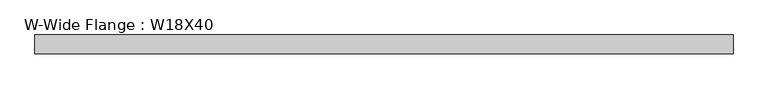
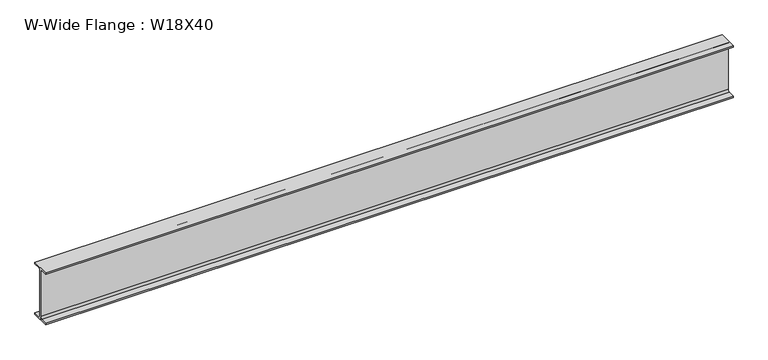
"""IFC4 building model written with IfcOpenShell, lengths in millimetres: beam geometry, W-Wide Flange : W18X40."""

from ifc_helpers import new_model, si_unit, point, frame, frame_2d, origin, place, context, project, spatial, polyline, circle_curve, trimmed, segment, composite_curve, outline, extrude, source, transform, mapped, element, save


def w_wide_flange_w18x40_c482f53b(model_context):
    return source(origin(), model_context, "Body", "SweptSolid", [
        extrude(outline(composite_curve([segment(polyline([(76.454, -213.995), (76.454, -227.33), (-76.454, -227.33), (-76.454, -213.995), (-20.828, -213.995)]), True, "CONTINUOUS"), segment(trimmed(circle_curve(frame_2d((-20.828, -197.1675)), 16.8275), [point((-20.828, -213.995))], [point((-4.0005, -197.1675))], True, "CARTESIAN"), True, "CONTINUOUS"), segment(polyline([(-4.0005, -197.1675), (-4.0005, 197.1675)]), True, "CONTINUOUS"), segment(trimmed(circle_curve(frame_2d((-20.828, 197.1675)), 16.8275), [point((-4.0005, 197.1675))], [point((-20.828, 213.995))], True, "CARTESIAN"), True, "CONTINUOUS"), segment(polyline([(-20.828, 213.995), (-76.454, 213.995), (-76.454, 227.33), (76.454, 227.33), (76.454, 213.995), (20.828, 213.995)]), True, "CONTINUOUS"), segment(trimmed(circle_curve(frame_2d((20.828, 197.1675)), 16.8275), [point((20.828, 213.995))], [point((4.0005, 197.1675))], True, "CARTESIAN"), True, "CONTINUOUS"), segment(polyline([(4.0005, 197.1675), (4.0005, -197.1675)]), True, "CONTINUOUS"), segment(trimmed(circle_curve(frame_2d((20.828, -197.1675)), 16.8275), [point((4.0005, -197.1675))], [point((20.828, -213.995))], True, "CARTESIAN"), True, "CONTINUOUS"), segment(polyline([(20.828, -213.995), (76.454, -213.995)]), True, "CONTINUOUS")], self_intersect=False)), frame((-2805.43, 0.0, 0.0), z_axis=(1.0, 0.0, 0.0), x_axis=(0.0, 1.0, 0.0)), (0.0, 0.0, 1.0), 5667.6925),
    ])


if __name__ == "__main__":
    model = new_model("IFC4")
    model_context = context("Model", 3, world=origin())
    ifc_project = project(units=[si_unit("LENGTHUNIT", "METRE", prefix="MILLI")], contexts=[model_context])
    site = spatial("IfcSite", under=ifc_project)
    building = spatial("IfcBuilding", under=site)
    placement = place(None, origin())
    w_wide_flange_w18x40_shape = w_wide_flange_w18x40_c482f53b(model_context)
    element("IfcBeam", 1, ObjectType="W-Wide Flange : W18X40", at=placement, inside=building, context=model_context, shape_type="MappedRepresentation", body=[
        mapped(w_wide_flange_w18x40_shape, transform((0.0, 0.0, 0.0), x_axis=(1.0, 0.0, 0.0), y_axis=(0.0, 1.0, 0.0), z_axis=(0.0, 0.0, 1.0))),
    ])
    save(model, "model.ifc")

# Revit data of these elements
# Type "W-Wide Flange : W18X40"
#   Assembly Code = "B10"
#   W = 40
#   Length [instance default] = 5' - 0"
#   bf = 0' - 6.02"
#   d = 1' - 5.9"
#   k = 0' - 1 3/16"
#   k2 = 0' - 0.6625"
#   tf = 0' - 0.525"
#   tw = 0' - 0.315"
#   A = 0.0819444 SF
#   Structural Material [instance default] = Steel ASTM A992
# Element 1 (IfcBeam, "W-Wide Flange : W18X40")
#   Materials on its faces: "Steel ASTM A992"
# Materials
#   "Steel ASTM A992": class "Metal", colour RGB 199 199 199, transparency 0, Description = "Structural steel 50ksi", Cost = 0
